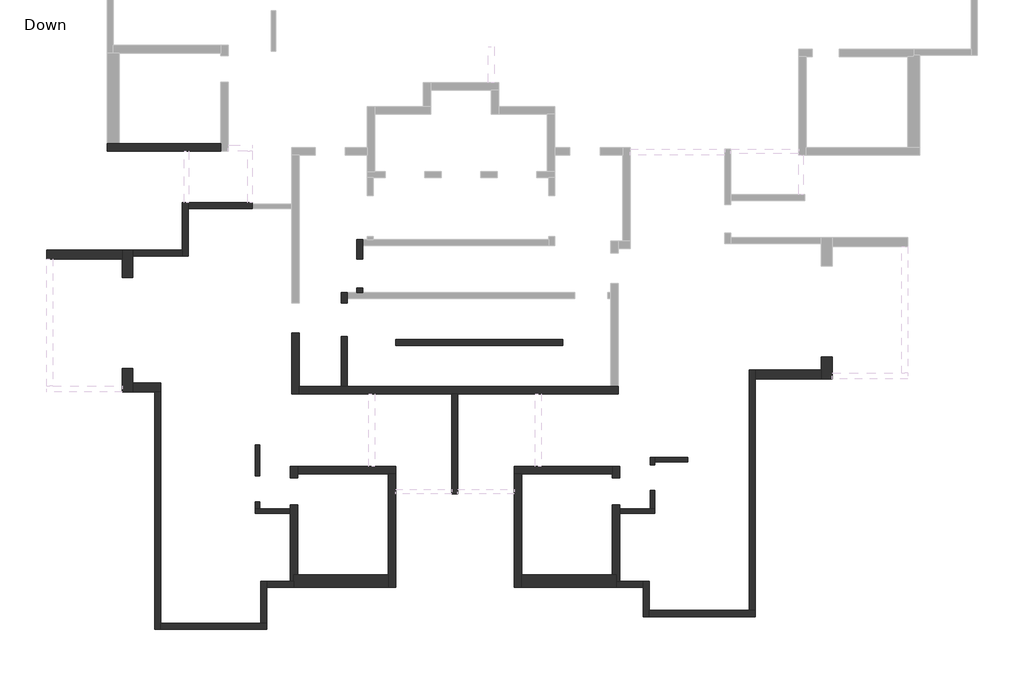
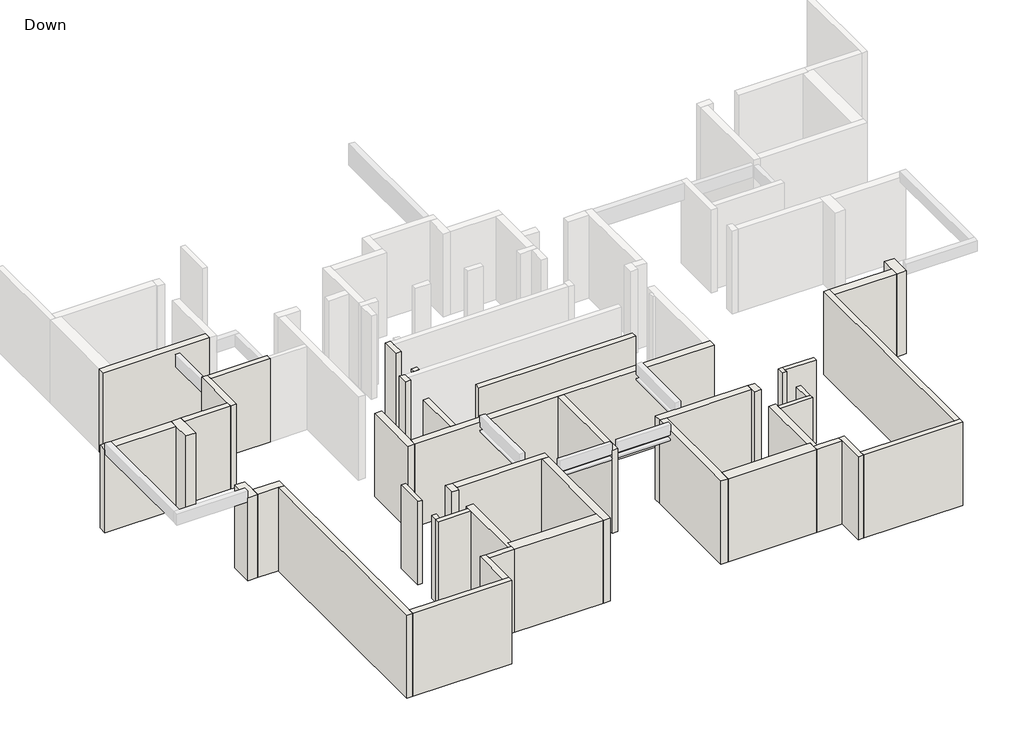
# One storey, part 1 of 3: 43 walls.
"""IFC4 building model written with IfcOpenShell, lengths in millimetres."""

import ifcopenshell
import ifcopenshell.guid

model = None  # the IFC model being written
_history = None  # IfcOwnerHistory: only IFC2X3 demands one
_inside = {}  # id of a spatial element -> (the spatial element, [elements in it])
_under = {}  # id of a project, library or spatial element -> (it, [spatial elements below it])
_declared = {}  # id of a project -> (the project, [libraries it declares])
_typed = {}  # id of a type object -> (the type object, [elements of that type])
_made_of = {}  # id of a material, layer set ... -> (it, [elements and type objects made of it])


def new_model(schema):
    """Start an empty IFC model of exactly this schema.

    Asked for "IFC4X3", IfcOpenShell would pick the latest addendum, in which some entities
    have other attributes; the version numbers below select the first issue.
    IFC2X3 requires an IfcOwnerHistory on every rooted entity: one is made here for all.
    """
    global model, _history
    if schema == "IFC4X3":
        model = ifcopenshell.file(schema_version=(4, 3, 0, 0))
    else:
        model = ifcopenshell.file(schema=schema)
    _inside.clear()
    _under.clear()
    _declared.clear()
    _typed.clear()
    _made_of.clear()
    _history = None
    if model.schema == "IFC2X3":
        org = make("IfcOrganization", Name="unknown")
        user = make(
            "IfcPersonAndOrganization",
            ThePerson=make("IfcPerson", FamilyName="unknown"),
            TheOrganization=org,
        )
        app = make(
            "IfcApplication",
            ApplicationDeveloper=org,
            Version="unknown",
            ApplicationFullName="unknown",
            ApplicationIdentifier="unknown",
        )
        _history = make(
            "IfcOwnerHistory",
            OwningUser=user,
            OwningApplication=app,
            ChangeAction="ADDED",
            CreationDate=0,
        )
    return model


def make(cls, **values):
    """One entity of the class cls with the attributes given. An attribute that is None is left unset."""
    return model.create_entity(
        cls, **{name: value for name, value in values.items() if value is not None}
    )


def rooted(cls, **values):
    """An entity with a GlobalId (a new one), such as an element, a storey or a relation."""
    return make(cls, GlobalId=ifcopenshell.guid.new(), OwnerHistory=_history, **values)


def si_unit(unit_type, name, prefix=None):
    """IfcSIUnit, for example si_unit("LENGTHUNIT", "METRE", prefix="MILLI")."""
    return make("IfcSIUnit", UnitType=unit_type, Prefix=prefix, Name=name)


def assignment(units):
    """IfcUnitAssignment: the units of a project."""
    return None if units is None else make("IfcUnitAssignment", Units=units)


def point(xyz):
    """IfcCartesianPoint."""
    return None if xyz is None else make("IfcCartesianPoint", Coordinates=xyz)


def direction(xyz):
    """IfcDirection."""
    return None if xyz is None else make("IfcDirection", DirectionRatios=xyz)


def frame(location, z_axis=None, x_axis=None):
    """IfcAxis2Placement3D, a coordinate frame: its origin and axes. An axis left out is left unset."""
    return make(
        "IfcAxis2Placement3D",
        Location=point(location),
        Axis=direction(z_axis),
        RefDirection=direction(x_axis),
    )


def origin():
    """The frame at (0, 0, 0) with its axes left unset."""
    return frame((0.0, 0.0, 0.0))


def place(relative_to, where):
    """IfcLocalPlacement: puts the frame where relative to a parent placement (None: the world)."""
    return make(
        "IfcLocalPlacement", PlacementRelTo=relative_to, RelativePlacement=where
    )


def context(
    kind, dimensions, precision=None, world=None, true_north=None, identifier=None
):
    """IfcGeometricRepresentationContext, for example the 3D "Model" context."""
    return make(
        "IfcGeometricRepresentationContext",
        ContextIdentifier=identifier,
        ContextType=kind,
        CoordinateSpaceDimension=dimensions,
        Precision=precision,
        WorldCoordinateSystem=world,
        TrueNorth=true_north,
    )


def project(units=None, contexts=None):
    """IfcProject with its units and contexts."""
    return rooted(
        "IfcProject",
        Name="project",
        RepresentationContexts=contexts,
        UnitsInContext=assignment(units),
    )


def spatial(cls, under=None, at=None, **own):
    """A site, building, storey or space (cls), placed at a placement, below another one or the project."""
    s = rooted(cls, ObjectPlacement=at, **own)
    if under is not None:
        _under.setdefault(under.id(), (under, []))[1].append(s)
    return s


def faces_of(points, faces, orient=None, outer=None):
    """IfcFace entities. A face is a list of loops; a loop is a list of indices into points, from 0.

    orient and outer hold one flag for each loop. By default every Orientation is true, the
    first loop of a face is its IfcFaceOuterBound and the others are IfcFaceBound.
    """
    made = []
    for i, loops in enumerate(faces):
        bounds = []
        for j, loop in enumerate(loops):
            is_outer = j == 0 if outer is None else outer[i][j]
            bounds.append(
                make(
                    "IfcFaceOuterBound" if is_outer else "IfcFaceBound",
                    Bound=make("IfcPolyLoop", Polygon=[points[k] for k in loop]),
                    Orientation=True if orient is None else orient[i][j],
                )
            )
        made.append(make("IfcFace", Bounds=bounds))
    return made


def faceted_brep(points, faces, orient=None, outer=None, voids=None):
    """IfcFacetedBrep: a solid bounded by flat faces; with voids (closed shells), ...WithVoids."""
    shared = [point(p) for p in points]
    hull = make("IfcClosedShell", CfsFaces=faces_of(shared, faces, orient, outer))
    if voids is None:
        return make("IfcFacetedBrep", Outer=hull)
    return make(
        "IfcFacetedBrepWithVoids",
        Outer=hull,
        Voids=[
            make(cls, CfsFaces=faces_of(shared, fs, o, b)) for cls, fs, o, b in voids
        ],
    )


def shape(context_of_items, identifier, shape_type, items):
    """IfcShapeRepresentation: the items that make up one representation, for example the "Body"."""
    return make(
        "IfcShapeRepresentation",
        ContextOfItems=context_of_items,
        RepresentationIdentifier=identifier,
        RepresentationType=shape_type,
        Items=items,
    )


def made_of(thing, what):
    """Note that an element or type object is made of a material, layer set ...; save() writes the relation."""
    if what is not None:
        _made_of.setdefault(what.id(), (what, []))[1].append(thing)
    return thing


def element(
    cls,
    number,
    at=None,
    inside=None,
    cuts=None,
    type_object=None,
    material=None,
    context=None,
    identifier="Body",
    shape_type=None,
    held_by="IfcProductDefinitionShape",
    body=None,
    shapes=None,
    **own,
):
    """One element of the class cls, such as IfcWall. Its Tag is "e" and its number.

    at: its placement. inside: the storey or other place that contains it. cuts: it is an
    opening in that element (IfcRelVoidsElement). A single representation is given by context,
    identifier, shape_type and body (its items); several are given by shapes. held_by: the class
    of the entity that holds the representations. save() writes the other relations.
    """
    e = rooted(cls, Tag="e%d" % number, ObjectPlacement=at, **own)
    if body is not None:
        shapes = [shape(context, identifier, shape_type, body)]
    if shapes is not None:
        e.Representation = make(held_by, Representations=shapes)
    if inside is not None:
        _inside.setdefault(inside.id(), (inside, []))[1].append(e)
    if cuts is not None:
        rooted(
            "IfcRelVoidsElement", RelatingBuildingElement=cuts, RelatedOpeningElement=e
        )
    if type_object is not None:
        _typed.setdefault(type_object.id(), (type_object, []))[1].append(e)
    return made_of(e, material)


def aggregate(whole, parts):
    """IfcRelAggregates: a whole, such as a stair, and the parts it consists of."""
    return rooted("IfcRelAggregates", RelatingObject=whole, RelatedObjects=parts)


def save(model, path):
    """Write the relations noted so far, then the file.

    IfcRelAggregates (storeys below a building ...), IfcRelContainedInSpatialStructure (elements
    in a storey), IfcRelDefinesByType, IfcRelAssociatesMaterial and IfcRelDeclares: one each for
    every whole, place, type object, material and project.
    """
    for whole, parts in _under.values():
        aggregate(whole, parts)
    for where, things in _inside.values():
        rooted(
            "IfcRelContainedInSpatialStructure",
            RelatedElements=things,
            RelatingStructure=where,
        )
    for kind, things in _typed.values():
        rooted("IfcRelDefinesByType", RelatedObjects=things, RelatingType=kind)
    for what, things in _made_of.values():
        rooted("IfcRelAssociatesMaterial", RelatedObjects=things, RelatingMaterial=what)
    for by, libraries in _declared.values():
        rooted("IfcRelDeclares", RelatingContext=by, RelatedDefinitions=libraries)
    model.write(path)


model = new_model("IFC4")

# Units and contexts
model_context = context("Model", 3, world=origin())
ifc_project = project(units=[si_unit("LENGTHUNIT", "METRE", prefix="MILLI")], contexts=[model_context])

# Site, building, storey
site = spatial("IfcSite", under=ifc_project)
building = spatial("IfcBuilding", under=site)
storey = spatial("IfcBuildingStorey", under=building, Name="Down", Elevation=0.0)

# Walls
placement = place(None, origin())
element("IfcWall", 1, ObjectType="15", at=placement, inside=storey, context=model_context, shape_type="Brep", body=[
    faceted_brep([(9202.7157481, -20705.5131366, 0.0), (8200.3527676, -20705.5131366, 0.0), (8050.3527676, -20705.5131366, 0.0), (8050.3527676, -20705.5131366, 3100.0), (8200.3527676, -20705.5131366, 3100.0), (9202.7157481, -20705.5131366, 3100.0), (9202.7157481, -20705.5131366, 2950.0), (9202.7157481, -20705.5131366, 2730.0), (9202.7157481, -20855.5131366, 0.0), (9202.7157481, -20855.5131366, 2730.0), (9202.7157481, -20855.5131366, 2950.0), (9202.7157481, -20855.5131366, 3100.0), (8050.3527676, -20855.5131366, 3100.0), (8050.3527676, -20855.5131366, 2950.0), (8050.3527676, -20855.5131366, 2730.0), (8050.3527676, -20855.5131366, 0.0)], [[[0, 1, 2, 3, 4, 5, 6, 7]], [[8, 9, 10, 11, 12, 13, 14, 15]], [[2, 1, 0, 8, 15]], [[5, 4, 3, 12, 11]], [[0, 7, 6, 5, 11, 10, 9, 8]], [[3, 2, 15, 14, 13, 12]]]),
])
element("IfcWall", 2, ObjectType="15", at=placement, inside=storey, context=model_context, shape_type="Brep", body=[
    faceted_brep([(8200.3527676, -20705.5131366, 0.0), (8200.3527676, -20474.3903326, 0.0), (8200.3527676, -20474.3903326, 2730.0), (8200.3527676, -20474.3903326, 2950.0), (8200.3527676, -20474.3903326, 3100.0), (8200.3527676, -20705.5131366, 3100.0), (8200.3527676, -20705.5131366, 2950.0), (8200.3527676, -20705.5131366, 2730.0), (8050.3527676, -20705.5131366, 0.0), (8050.3527676, -20705.5131366, 3100.0), (8050.3527676, -20474.3903326, 3100.0), (8050.3527676, -20474.3903326, 2950.0), (8050.3527676, -20474.3903326, 2730.0), (8050.3527676, -20474.3903326, 0.0)], [[[0, 1, 2, 3, 4, 5, 6, 7]], [[8, 9, 10, 11, 12, 13]], [[1, 0, 8, 13]], [[4, 3, 2, 1, 13, 12, 11, 10]], [[5, 4, 10, 9]], [[0, 7, 6, 5, 9, 8]]]),
])
element("IfcWall", 3, ObjectType="15", at=placement, inside=storey, context=model_context, shape_type="Brep", body=[
    faceted_brep([(8200.3527676, -19623.2572222, 0.0), (8200.3527676, -18603.3436751, 0.0), (8200.3527676, -18603.3436751, 2730.0), (8200.3527676, -18603.3436751, 2950.0), (8200.3527676, -18603.3436751, 3100.0), (8200.3527676, -19623.2572222, 3100.0), (8200.3527676, -19623.2572222, 2950.0), (8200.3527676, -19623.2572222, 2730.0), (8050.3527676, -19623.2572222, 0.0), (8050.3527676, -19623.2572222, 2730.0), (8050.3527676, -19623.2572222, 2950.0), (8050.3527676, -19623.2572222, 3100.0), (8050.3527676, -18603.3436751, 3100.0), (8050.3527676, -18603.3436751, 2950.0), (8050.3527676, -18603.3436751, 2730.0), (8050.3527676, -18603.3436751, 0.0)], [[[0, 1, 2, 3, 4, 5, 6, 7]], [[8, 9, 10, 11, 12, 13, 14, 15]], [[1, 0, 8, 15]], [[4, 3, 2, 1, 15, 14, 13, 12]], [[5, 4, 12, 11]], [[0, 7, 6, 5, 11, 10, 9, 8]]]),
])
element("IfcWall", 4, ObjectType="15", at=placement, inside=storey, context=model_context, shape_type="Brep", body=[
    faceted_brep([(20111.1907174, -20855.5131366, 0.0), (21263.5536979, -20855.5131366, 0.0), (21263.5536979, -20855.5131366, 2730.0), (21263.5536979, -20855.5131366, 2950.0), (21263.5536979, -20855.5131366, 3100.0), (20111.1907174, -20855.5131366, 3100.0), (20111.1907174, -20855.5131366, 2950.0), (20111.1907174, -20855.5131366, 2730.0), (20111.1907174, -20705.5131366, 0.0), (20111.1907174, -20705.5131366, 2730.0), (20111.1907174, -20705.5131366, 2950.0), (20111.1907174, -20705.5131366, 3100.0), (21113.5536979, -20705.5131366, 3100.0), (21263.5536979, -20705.5131366, 3100.0), (21263.5536979, -20705.5131366, 0.0), (21113.5536979, -20705.5131366, 0.0)], [[[0, 1, 2, 3, 4, 5, 6, 7]], [[8, 9, 10, 11, 12, 13, 14, 15]], [[1, 0, 8, 15, 14]], [[5, 4, 13, 12, 11]], [[0, 7, 6, 5, 11, 10, 9, 8]], [[4, 3, 2, 1, 14, 13]]]),
])
element("IfcWall", 5, ObjectType="15", at=placement, inside=storey, context=model_context, shape_type="Brep", body=[
    faceted_brep([(21263.5536979, -20705.5131366, 0.0), (21263.5536979, -20105.5131366, 0.0), (21263.5536979, -20105.5131366, 2730.0), (21263.5536979, -20105.5131366, 2950.0), (21263.5536979, -20105.5131366, 3100.0), (21263.5536979, -20705.5131366, 3100.0), (21113.5536979, -20705.5131366, 0.0), (21113.5536979, -20705.5131366, 2730.0), (21113.5536979, -20705.5131366, 2950.0), (21113.5536979, -20705.5131366, 3100.0), (21113.5536979, -20105.5131366, 3100.0), (21113.5536979, -20105.5131366, 2950.0), (21113.5536979, -20105.5131366, 2730.0), (21113.5536979, -20105.5131366, 0.0)], [[[0, 1, 2, 3, 4, 5]], [[6, 7, 8, 9, 10, 11, 12, 13]], [[1, 0, 6, 13]], [[4, 3, 2, 1, 13, 12, 11, 10]], [[5, 4, 10, 9]], [[0, 5, 9, 8, 7, 6]]]),
])
element("IfcWall", 6, ObjectType="15", at=placement, inside=storey, context=model_context, shape_type="Brep", body=[
    faceted_brep([(21258.5265415, -19255.7144534, 0.0), (21258.5265415, -19155.8065343, 0.0), (21258.5265415, -19005.8065343, 0.0), (21258.5265415, -19005.8065343, 3100.0), (21258.5265415, -19155.8065343, 3100.0), (21258.5265415, -19255.7144534, 3100.0), (21258.5265415, -19255.7144534, 2950.0), (21258.5265415, -19255.7144534, 2730.0), (21108.5265415, -19255.7144534, 0.0), (21108.5265415, -19255.7144534, 2730.0), (21108.5265415, -19255.7144534, 2950.0), (21108.5265415, -19255.7144534, 3100.0), (21108.5265415, -19005.8065343, 3100.0), (21108.5265415, -19005.8065343, 2950.0), (21108.5265415, -19005.8065343, 2730.0), (21108.5265415, -19005.8065343, 0.0)], [[[0, 1, 2, 3, 4, 5, 6, 7]], [[8, 9, 10, 11, 12, 13, 14, 15]], [[2, 1, 0, 8, 15]], [[5, 4, 3, 12, 11]], [[0, 7, 6, 5, 11, 10, 9, 8]], [[3, 2, 15, 14, 13, 12]]]),
])
element("IfcWall", 7, ObjectType="15", at=placement, inside=storey, context=model_context, shape_type="Brep", body=[
    faceted_brep([(21258.5265415, -19155.8065343, 0.0), (22357.1843165, -19155.8065343, 0.0), (22357.1843165, -19155.8065343, 2730.0), (22357.1843165, -19155.8065343, 2950.0), (22357.1843165, -19155.8065343, 3100.0), (21258.5265415, -19155.8065343, 3100.0), (21258.5265415, -19155.8065343, 2950.0), (21258.5265415, -19155.8065343, 2730.0), (21258.5265415, -19005.8065343, 0.0), (21258.5265415, -19005.8065343, 3100.0), (22357.1843165, -19005.8065343, 3100.0), (22357.1843165, -19005.8065343, 2950.0), (22357.1843165, -19005.8065343, 2730.0), (22357.1843165, -19005.8065343, 0.0)], [[[0, 1, 2, 3, 4, 5, 6, 7]], [[8, 9, 10, 11, 12, 13]], [[1, 0, 8, 13]], [[4, 3, 2, 1, 13, 12, 11, 10]], [[5, 4, 10, 9]], [[0, 7, 6, 5, 9, 8]]]),
])
element("IfcWall", 8, ObjectType="20", at=placement, inside=storey, context=model_context, shape_type="Brep", body=[
    faceted_brep([(4004.7368494, -12353.0033555, 0.0), (5645.6252471, -12353.0033555, 0.0), (5645.6252471, -12353.0033555, 3100.0), (4004.7368494, -12353.0033555, 3100.0), (4004.7368494, -12353.0033555, 2950.0), (4004.7368494, -12353.0033555, 2730.0), (4004.7368494, -12153.0033555, 0.0), (4004.7368494, -12153.0033555, 3100.0), (5645.6252471, -12153.0033555, 3100.0), (5645.6252471, -12153.0033555, 0.0)], [[[0, 1, 2, 3, 4, 5]], [[6, 7, 8, 9]], [[1, 0, 6, 9]], [[3, 2, 8, 7]], [[2, 1, 9, 8]], [[0, 5, 4, 3, 7, 6]]]),
])
element("IfcWall", 9, ObjectType="20", at=placement, inside=storey, context=model_context, shape_type="Brep", body=[
    faceted_brep([(5845.6252471, -12353.0033555, 0.0), (5845.6252471, -10774.5447275, 0.0), (5845.6252471, -10574.5447275, 0.0), (5845.6252471, -10574.5447275, 3100.0), (5845.6252471, -10774.5447275, 3100.0), (5845.6252471, -12353.0033555, 3100.0), (5845.6252471, -12353.0033555, 2950.0), (5845.6252471, -12353.0033555, 2730.0), (5645.6252471, -12353.0033555, 0.0), (5645.6252471, -12353.0033555, 3100.0), (5645.6252471, -12153.0033555, 3100.0), (5645.6252471, -10574.5447275, 3100.0), (5645.6252471, -10574.5447275, 0.0), (5645.6252471, -12153.0033555, 0.0)], [[[0, 1, 2, 3, 4, 5, 6, 7]], [[8, 9, 10, 11, 12, 13]], [[2, 1, 0, 8, 13, 12]], [[5, 4, 3, 11, 10, 9]], [[0, 7, 6, 5, 9, 8]], [[3, 2, 12, 11]]]),
])
element("IfcWall", 10, ObjectType="20", at=placement, inside=storey, context=model_context, shape_type="Brep", body=[
    faceted_brep([(5845.6252471, -10774.5447275, 0.0), (7954.0579731, -10774.5447275, 0.0), (7954.0579731, -10774.5447275, 3100.0), (5845.6252471, -10774.5447275, 3100.0), (5845.6252471, -10774.5447275, 2950.0), (5845.6252471, -10774.5447275, 2730.0), (5845.6252471, -10574.5447275, 0.0), (5845.6252471, -10574.5447275, 3100.0), (7954.0579731, -10574.5447275, 3100.0), (7954.0579731, -10574.5447275, 2450.0), (7954.0579731, -10574.5447275, 2300.0), (7954.0579731, -10574.5447275, 0.0), (7954.0579731, -10624.5447275, 0.0), (7954.0579731, -10624.5447275, 3100.0)], [[[0, 1, 2, 3, 4, 5]], [[6, 7, 8, 9, 10, 11]], [[1, 0, 6, 11, 12]], [[2, 1, 12, 11, 10, 9, 8, 13]], [[3, 2, 13, 8, 7]], [[0, 5, 4, 3, 7, 6]]]),
])
element("IfcWall", 11, ObjectType="20", at=placement, inside=storey, context=model_context, shape_type="Brep", body=[
    faceted_brep([(4732.0592479, -16842.3482114, 0.0), (4732.0592479, -24693.724882, 0.0), (4732.0592479, -24693.724882, 3100.0), (4732.0592479, -16842.3482114, 3100.0), (4932.0592479, -16842.3482114, 0.0), (4932.0592479, -16842.3482114, 3100.0), (4932.0592479, -24493.724882, 3100.0), (4932.0592479, -24693.724882, 3100.0), (4932.0592479, -24693.724882, 0.0), (4932.0592479, -24493.724882, 0.0)], [[[0, 1, 2, 3]], [[4, 5, 6, 7, 8, 9]], [[1, 0, 4, 9, 8]], [[3, 2, 7, 6, 5]], [[2, 1, 8, 7]], [[0, 3, 5, 4]]]),
])
element("IfcWall", 12, ObjectType="20", at=placement, inside=storey, context=model_context, shape_type="Brep", body=[
    faceted_brep([(4932.0592479, -24693.724882, 0.0), (8431.4755716, -24693.724882, 0.0), (8431.4755716, -24693.724882, 3100.0), (4932.0592479, -24693.724882, 3100.0), (4932.0592479, -24493.724882, 0.0), (4932.0592479, -24493.724882, 2730.0), (4932.0592479, -24493.724882, 2950.0), (4932.0592479, -24493.724882, 3100.0), (8231.4755716, -24493.724882, 3100.0), (8431.4755716, -24493.724882, 3100.0), (8431.4755716, -24493.724882, 0.0), (8231.4755716, -24493.724882, 0.0)], [[[0, 1, 2, 3]], [[4, 5, 6, 7, 8, 9, 10, 11]], [[1, 0, 4, 11, 10]], [[3, 2, 9, 8, 7]], [[0, 3, 7, 6, 5, 4]], [[2, 1, 10, 9]]]),
])
element("IfcWall", 13, ObjectType="20", at=placement, inside=storey, context=model_context, shape_type="Brep", body=[
    faceted_brep([(8431.4755716, -24493.724882, 0.0), (8431.4755716, -23302.7444034, 0.0), (8431.4755716, -23102.7444034, 0.0), (8431.4755716, -23102.7444034, 3100.0), (8431.4755716, -23302.7444034, 3100.0), (8431.4755716, -24493.724882, 3100.0), (8231.4755716, -24493.724882, 0.0), (8231.4755716, -24493.724882, 2730.0), (8231.4755716, -24493.724882, 2950.0), (8231.4755716, -24493.724882, 3100.0), (8231.4755716, -23102.7444034, 3100.0), (8231.4755716, -23102.7444034, 2950.0), (8231.4755716, -23102.7444034, 2730.0), (8231.4755716, -23102.7444034, 0.0)], [[[0, 1, 2, 3, 4, 5]], [[6, 7, 8, 9, 10, 11, 12, 13]], [[2, 1, 0, 6, 13]], [[5, 4, 3, 10, 9]], [[0, 5, 9, 8, 7, 6]], [[3, 2, 13, 12, 11, 10]]]),
])
element("IfcWall", 14, ObjectType="20", at=placement, inside=storey, context=model_context, shape_type="Brep", body=[
    faceted_brep([(8431.4755716, -23302.7444034, 0.0), (9327.7157481, -23302.7444034, 0.0), (9327.7157481, -23302.7444034, 3100.0), (8431.4755716, -23302.7444034, 3100.0), (8431.4755716, -23102.7444034, 0.0), (8431.4755716, -23102.7444034, 3100.0), (9202.7157481, -23102.7444034, 3100.0), (9327.7157481, -23102.7444034, 3100.0), (9327.7157481, -23102.7444034, 0.0), (9202.7157481, -23102.7444034, 0.0)], [[[0, 1, 2, 3]], [[4, 5, 6, 7, 8, 9]], [[1, 0, 4, 9, 8]], [[2, 1, 8, 7]], [[3, 2, 7, 6, 5]], [[0, 3, 5, 4]]]),
])
element("IfcWall", 15, ObjectType="20", at=placement, inside=storey, context=model_context, shape_type="Brep", body=[
    faceted_brep([(14756.9532328, -20224.3060494, 0.0), (14756.9532328, -16906.0156488, 0.0), (14756.9532328, -16906.0156488, 2800.0), (14756.9532328, -16906.0156488, 2950.0), (14756.9532328, -16906.0156488, 3100.0), (14756.9532328, -20224.3060494, 3100.0), (14756.9532328, -20224.3060494, 2950.0), (14756.9532328, -20224.3060494, 2800.0), (14756.9532328, -20224.3060494, 2750.0), (14556.9532328, -20224.3060494, 0.0), (14556.9532328, -20224.3060494, 2750.0), (14556.9532328, -20224.3060494, 2800.0), (14556.9532328, -20224.3060494, 2950.0), (14556.9532328, -20224.3060494, 3100.0), (14556.9532328, -16906.0156488, 3100.0), (14556.9532328, -16906.0156488, 2950.0), (14556.9532328, -16906.0156488, 2800.0), (14556.9532328, -16906.0156488, 0.0)], [[[0, 1, 2, 3, 4, 5, 6, 7, 8]], [[9, 10, 11, 12, 13, 14, 15, 16, 17]], [[1, 0, 9, 17]], [[5, 4, 14, 13]], [[0, 8, 7, 6, 5, 13, 12, 11, 10, 9]], [[4, 3, 2, 1, 17, 16, 15, 14]]]),
])
element("IfcWall", 16, ObjectType="20", at=placement, inside=storey, context=model_context, shape_type="Brep", body=[
    faceted_brep([(21082.430894, -24277.7444034, 0.0), (21082.430894, -24077.7444034, 0.0), (21082.430894, -23102.7444034, 0.0), (21082.430894, -23102.7444034, 2730.0), (21082.430894, -23102.7444034, 2950.0), (21082.430894, -23102.7444034, 3100.0), (21082.430894, -24077.7444034, 3100.0), (21082.430894, -24277.7444034, 3100.0), (20882.430894, -24277.7444034, 0.0), (20882.430894, -24277.7444034, 3100.0), (20882.430894, -23302.7444034, 3100.0), (20882.430894, -23102.7444034, 3100.0), (20882.430894, -23102.7444034, 0.0), (20882.430894, -23302.7444034, 0.0)], [[[0, 1, 2, 3, 4, 5, 6, 7]], [[8, 9, 10, 11, 12, 13]], [[2, 1, 0, 8, 13, 12]], [[7, 6, 5, 11, 10, 9]], [[5, 4, 3, 2, 12, 11]], [[0, 7, 9, 8]]]),
])
element("IfcWall", 17, ObjectType="20", at=placement, inside=storey, context=model_context, shape_type="Brep", body=[
    faceted_brep([(20882.430894, -23102.7444034, 0.0), (20111.1907174, -23102.7444034, 0.0), (19986.1907174, -23102.7444034, 0.0), (19986.1907174, -23102.7444034, 3100.0), (20111.1907174, -23102.7444034, 3100.0), (20882.430894, -23102.7444034, 3100.0), (20882.430894, -23302.7444034, 0.0), (20882.430894, -23302.7444034, 3100.0), (19986.1907174, -23302.7444034, 3100.0), (19986.1907174, -23302.7444034, 0.0)], [[[0, 1, 2, 3, 4, 5]], [[6, 7, 8, 9]], [[2, 1, 0, 6, 9]], [[3, 2, 9, 8]], [[5, 4, 3, 8, 7]], [[0, 5, 7, 6]]]),
])
element("IfcWall", 18, ObjectType="20", at=placement, inside=storey, context=model_context, shape_type="Brep", body=[
    faceted_brep([(21082.430894, -24277.7444034, 0.0), (24582.430894, -24277.7444034, 0.0), (24582.430894, -24277.7444034, 3100.0), (21082.430894, -24277.7444034, 3100.0), (21082.430894, -24077.7444034, 0.0), (21082.430894, -24077.7444034, 2730.0), (21082.430894, -24077.7444034, 2950.0), (21082.430894, -24077.7444034, 3100.0), (24382.430894, -24077.7444034, 3100.0), (24582.430894, -24077.7444034, 3100.0), (24582.430894, -24077.7444034, 0.0), (24382.430894, -24077.7444034, 0.0)], [[[0, 1, 2, 3]], [[4, 5, 6, 7, 8, 9, 10, 11]], [[1, 0, 4, 11, 10]], [[3, 2, 9, 8, 7]], [[0, 3, 7, 6, 5, 4]], [[2, 1, 10, 9]]]),
])
element("IfcWall", 19, ObjectType="20", at=placement, inside=storey, context=model_context, shape_type="Brep", body=[
    faceted_brep([(24582.430894, -24077.7444034, 0.0), (24582.430894, -16418.7263398, 0.0), (24582.430894, -16118.7263398, 0.0), (24582.430894, -16118.7263398, 3100.0), (24582.430894, -16418.7263398, 3100.0), (24582.430894, -24077.7444034, 3100.0), (24382.430894, -24077.7444034, 0.0), (24382.430894, -24077.7444034, 2730.0), (24382.430894, -24077.7444034, 2950.0), (24382.430894, -24077.7444034, 3100.0), (24382.430894, -16118.7263398, 3100.0), (24382.430894, -16118.7263398, 2950.0), (24382.430894, -16118.7263398, 2730.0), (24382.430894, -16118.7263398, 0.0)], [[[0, 1, 2, 3, 4, 5]], [[6, 7, 8, 9, 10, 11, 12, 13]], [[2, 1, 0, 6, 13]], [[5, 4, 3, 10, 9]], [[0, 5, 9, 8, 7, 6]], [[3, 2, 13, 12, 11, 10]]]),
])
element("IfcWall", 20, ObjectType="20", at=placement, inside=storey, context=model_context, shape_type="Brep", body=[
    faceted_brep([(11403.5632586, -11804.3284255, 0.0), (11403.5632586, -12452.9986769, 0.0), (11403.5632586, -12452.9986769, 2730.0), (11403.5632586, -12452.9986769, 2950.0), (11403.5632586, -12452.9986769, 3100.0), (11403.5632586, -11804.3284255, 3100.0), (11403.5632586, -11804.3284255, 2950.0), (11403.5632586, -11804.3284255, 2730.0), (11603.5632586, -11804.3284255, 0.0), (11603.5632586, -11804.3284255, 3100.0), (11603.5632586, -12004.3284255, 3100.0), (11603.5632586, -12452.9986769, 3100.0), (11603.5632586, -12452.9986769, 2950.0), (11603.5632586, -12452.9986769, 2730.0), (11603.5632586, -12452.9986769, 0.0), (11603.5632586, -12004.3284255, 0.0)], [[[0, 1, 2, 3, 4, 5, 6, 7]], [[8, 9, 10, 11, 12, 13, 14, 15]], [[1, 0, 8, 15, 14]], [[4, 3, 2, 1, 14, 13, 12, 11]], [[5, 4, 11, 10, 9]], [[0, 7, 6, 5, 9, 8]]]),
])
element("IfcWall", 21, ObjectType="20", at=placement, inside=storey, context=model_context, shape_type="Brep", body=[
    faceted_brep([(11403.5632586, -13405.3647765, 0.0), (11403.5632586, -13552.8020387, 0.0), (11403.5632586, -13552.8020387, 2730.0), (11403.5632586, -13552.8020387, 2950.0), (11403.5632586, -13552.8020387, 3100.0), (11403.5632586, -13405.3647765, 3100.0), (11403.5632586, -13405.3647765, 2950.0), (11403.5632586, -13405.3647765, 2730.0), (11603.5632586, -13405.3647765, 0.0), (11603.5632586, -13405.3647765, 2730.0), (11603.5632586, -13405.3647765, 2950.0), (11603.5632586, -13405.3647765, 3100.0), (11603.5632586, -13552.8020387, 3100.0), (11603.5632586, -13552.8020387, 2950.0), (11603.5632586, -13552.8020387, 2730.0), (11603.5632586, -13552.8020387, 0.0)], [[[0, 1, 2, 3, 4, 5, 6, 7]], [[8, 9, 10, 11, 12, 13, 14, 15]], [[1, 0, 8, 15]], [[5, 4, 12, 11]], [[0, 7, 6, 5, 11, 10, 9, 8]], [[4, 3, 2, 1, 15, 14, 13, 12]]]),
])
element("IfcWall", 22, ObjectType="20", at=placement, inside=storey, context=model_context, shape_type="Brep", body=[
    faceted_brep([(10900.0437745, -13552.8020387, 0.0), (10900.0437745, -13905.1806146, 0.0), (10900.0437745, -13905.1806146, 2730.0), (10900.0437745, -13905.1806146, 2950.0), (10900.0437745, -13905.1806146, 3100.0), (10900.0437745, -13552.8020387, 3100.0), (10900.0437745, -13552.8020387, 2950.0), (10900.0437745, -13552.8020387, 2730.0), (11100.0437745, -13552.8020387, 0.0), (11100.0437745, -13552.8020387, 3100.0), (11100.0437745, -13752.8020387, 3100.0), (11100.0437745, -13905.1806146, 3100.0), (11100.0437745, -13905.1806146, 2950.0), (11100.0437745, -13905.1806146, 2730.0), (11100.0437745, -13905.1806146, 0.0), (11100.0437745, -13752.8020387, 0.0)], [[[0, 1, 2, 3, 4, 5, 6, 7]], [[8, 9, 10, 11, 12, 13, 14, 15]], [[1, 0, 8, 15, 14]], [[4, 3, 2, 1, 14, 13, 12, 11]], [[5, 4, 11, 10, 9]], [[0, 7, 6, 5, 9, 8]]]),
])
element("IfcWall", 23, ObjectType="20", at=placement, inside=storey, context=model_context, shape_type="Brep", body=[
    faceted_brep([(10900.0437745, -15005.1634597, 0.0), (10900.0437745, -16656.0156488, 0.0), (10900.0437745, -16656.0156488, 2730.0), (10900.0437745, -16656.0156488, 2950.0), (10900.0437745, -16656.0156488, 3100.0), (10900.0437745, -15005.1634597, 3100.0), (10900.0437745, -15005.1634597, 2950.0), (10900.0437745, -15005.1634597, 2730.0), (11100.0437745, -15005.1634597, 0.0), (11100.0437745, -15005.1634597, 2730.0), (11100.0437745, -15005.1634597, 2950.0), (11100.0437745, -15005.1634597, 3100.0), (11100.0437745, -16656.0156488, 3100.0), (11100.0437745, -16656.0156488, 2950.0), (11100.0437745, -16656.0156488, 2730.0), (11100.0437745, -16656.0156488, 0.0)], [[[0, 1, 2, 3, 4, 5, 6, 7]], [[8, 9, 10, 11, 12, 13, 14, 15]], [[1, 0, 8, 15]], [[5, 4, 12, 11]], [[0, 7, 6, 5, 11, 10, 9, 8]], [[4, 3, 2, 1, 15, 14, 13, 12]]]),
])
element("IfcWall", 24, ObjectType="20", at=placement, inside=storey, context=model_context, shape_type="Brep", body=[
    faceted_brep([(12694.7247799, -15306.2169656, 0.0), (18213.8626911, -15306.2169656, 0.0), (18213.8626911, -15306.2169656, 2730.0), (18213.8626911, -15306.2169656, 2950.0), (18213.8626911, -15306.2169656, 3100.0), (12694.7247799, -15306.2169656, 3100.0), (12694.7247799, -15106.2169656, 0.0), (12694.7247799, -15106.2169656, 3100.0), (18213.8626911, -15106.2169656, 3100.0), (18213.8626911, -15106.2169656, 2950.0), (18213.8626911, -15106.2169656, 2730.0), (18213.8626911, -15106.2169656, 0.0)], [[[0, 1, 2, 3, 4, 5]], [[6, 7, 8, 9, 10, 11]], [[1, 0, 6, 11]], [[4, 3, 2, 1, 11, 10, 9, 8]], [[5, 4, 8, 7]], [[0, 5, 7, 6]]]),
])
element("IfcWall", 25, ObjectType="25", at=placement, inside=storey, context=model_context, shape_type="Brep", body=[
    faceted_brep([(6907.9504595, -8625.9821525, 0.0), (3557.3073849, -8625.9821525, 0.0), (3157.3073849, -8625.9821525, 0.0), (3157.3073849, -8625.9821525, 3100.0), (3557.3073849, -8625.9821525, 3100.0), (6907.9504595, -8625.9821525, 3100.0), (6907.9504595, -8625.9821525, 2950.0), (6907.9504595, -8625.9821525, 2730.0), (6907.9504595, -8875.9821525, 0.0), (6907.9504595, -8875.9821525, 3100.0), (3157.3073849, -8875.9821525, 3100.0), (3157.3073849, -8875.9821525, 0.0)], [[[0, 1, 2, 3, 4, 5, 6, 7]], [[8, 9, 10, 11]], [[2, 1, 0, 8, 11]], [[5, 4, 3, 10, 9]], [[0, 7, 6, 5, 9, 8]], [[3, 2, 11, 10]]]),
])
element("IfcWall", 26, ObjectType="25", at=placement, inside=storey, context=model_context, shape_type="Brep", body=[
    faceted_brep([(9452.7157481, -19695.7428642, 0.0), (9452.7157481, -19551.9218456, 0.0), (9452.7157481, -19301.9218456, 0.0), (9452.7157481, -19301.9218456, 3100.0), (9452.7157481, -19551.9218456, 3100.0), (9452.7157481, -19695.7428642, 3100.0), (9452.7157481, -19695.7428642, 2950.0), (9452.7157481, -19695.7428642, 2730.0), (9202.7157481, -19695.7428642, 0.0), (9202.7157481, -19695.7428642, 2730.0), (9202.7157481, -19695.7428642, 2950.0), (9202.7157481, -19695.7428642, 3100.0), (9202.7157481, -19301.9218456, 3100.0), (9202.7157481, -19301.9218456, 2950.0), (9202.7157481, -19301.9218456, 2730.0), (9202.7157481, -19301.9218456, 0.0)], [[[0, 1, 2, 3, 4, 5, 6, 7]], [[8, 9, 10, 11, 12, 13, 14, 15]], [[2, 1, 0, 8, 15]], [[5, 4, 3, 12, 11]], [[0, 7, 6, 5, 11, 10, 9, 8]], [[3, 2, 15, 14, 13, 12]]]),
])
element("IfcWall", 27, ObjectType="25", at=placement, inside=storey, context=model_context, shape_type="Brep", body=[
    faceted_brep([(9452.7157481, -19551.9218456, 0.0), (12452.1320718, -19551.9218456, 0.0), (12702.1320718, -19551.9218456, 0.0), (12702.1320718, -19551.9218456, 3100.0), (12452.1320718, -19551.9218456, 3100.0), (9452.7157481, -19551.9218456, 3100.0), (9452.7157481, -19551.9218456, 2950.0), (9452.7157481, -19551.9218456, 2730.0), (9452.7157481, -19301.9218456, 0.0), (9452.7157481, -19301.9218456, 3100.0), (12702.1320718, -19301.9218456, 3100.0), (12702.1320718, -19301.9218456, 2950.0), (12702.1320718, -19301.9218456, 2800.0), (12702.1320718, -19301.9218456, 0.0)], [[[0, 1, 2, 3, 4, 5, 6, 7]], [[8, 9, 10, 11, 12, 13]], [[2, 1, 0, 8, 13]], [[5, 4, 3, 10, 9]], [[0, 7, 6, 5, 9, 8]], [[3, 2, 13, 12, 11, 10]]]),
])
element("IfcWall", 28, ObjectType="25", at=placement, inside=storey, context=model_context, shape_type="Brep", body=[
    faceted_brep([(12452.1320718, -19551.9218456, 0.0), (12452.1320718, -22902.7444034, 0.0), (12452.1320718, -23302.7444034, 0.0), (12452.1320718, -23302.7444034, 3100.0), (12452.1320718, -22902.7444034, 3100.0), (12452.1320718, -19551.9218456, 3100.0), (12452.1320718, -19551.9218456, 2950.0), (12452.1320718, -19551.9218456, 2730.0), (12702.1320718, -19551.9218456, 0.0), (12702.1320718, -19551.9218456, 3100.0), (12702.1320718, -23302.7444034, 3100.0), (12702.1320718, -23302.7444034, 0.0)], [[[0, 1, 2, 3, 4, 5, 6, 7]], [[8, 9, 10, 11]], [[2, 1, 0, 8, 11]], [[5, 4, 3, 10, 9]], [[0, 7, 6, 5, 9, 8]], [[3, 2, 11, 10]]]),
])
element("IfcWall", 29, ObjectType="25", at=placement, inside=storey, context=model_context, shape_type="Brep", body=[
    faceted_brep([(9452.7157481, -22902.7444034, 0.0), (9452.7157481, -20584.2651623, 0.0), (9452.7157481, -20584.2651623, 2730.0), (9452.7157481, -20584.2651623, 2950.0), (9452.7157481, -20584.2651623, 3100.0), (9452.7157481, -22902.7444034, 3100.0), (9452.7157481, -22902.7444034, 2950.0), (9452.7157481, -22902.7444034, 2730.0), (9202.7157481, -23102.7444034, 0.0), (9202.7157481, -23102.7444034, 2730.0), (9202.7157481, -23102.7444034, 2950.0), (9202.7157481, -23102.7444034, 3100.0), (9202.7157481, -20855.5131366, 3100.0), (9202.7157481, -20705.5131366, 3100.0), (9202.7157481, -20584.2651623, 3100.0), (9202.7157481, -20584.2651623, 2950.0), (9202.7157481, -20584.2651623, 2730.0), (9202.7157481, -20584.2651623, 0.0), (9202.7157481, -20705.5131366, 0.0), (9202.7157481, -20855.5131366, 0.0), (9327.7157481, -22902.7444034, 0.0), (9327.7157481, -23102.7444034, 0.0), (9327.7157481, -23102.7444034, 3100.0), (9327.7157481, -22902.7444034, 3100.0)], [[[0, 1, 2, 3, 4, 5, 6, 7]], [[8, 9, 10, 11, 12, 13, 14, 15, 16, 17, 18, 19]], [[1, 0, 20, 21, 8, 19, 18, 17]], [[4, 3, 2, 1, 17, 16, 15, 14]], [[5, 4, 14, 13, 12, 11, 22, 23]], [[0, 7, 6, 5, 23, 20]], [[23, 22, 21, 20]], [[22, 11, 10, 9, 8, 21]]]),
])
element("IfcWall", 30, ObjectType="25", at=placement, inside=storey, context=model_context, shape_type="Brep", body=[
    faceted_brep([(9252.7110695, -14895.1122659, 0.0), (9252.7110695, -16906.0156488, 0.0), (9252.7110695, -16906.0156488, 2730.0), (9252.7110695, -16906.0156488, 2950.0), (9252.7110695, -16906.0156488, 3100.0), (9252.7110695, -14895.1122659, 3100.0), (9502.7110695, -14895.1122659, 0.0), (9502.7110695, -14895.1122659, 3100.0), (9502.7110695, -16656.0156488, 3100.0), (9502.7110695, -16906.0156488, 3100.0), (9502.7110695, -16906.0156488, 0.0), (9502.7110695, -16656.0156488, 0.0)], [[[0, 1, 2, 3, 4, 5]], [[6, 7, 8, 9, 10, 11]], [[1, 0, 6, 11, 10]], [[5, 4, 9, 8, 7]], [[0, 5, 7, 6]], [[4, 3, 2, 1, 10, 9]]]),
])
element("IfcWall", 31, ObjectType="25", at=placement, inside=storey, context=model_context, shape_type="Brep", body=[
    faceted_brep([(9502.7110695, -16906.0156488, 0.0), (14556.9532328, -16906.0156488, 0.0), (14756.9532328, -16906.0156488, 0.0), (20058.6310988, -16906.0156488, 0.0), (20058.6310988, -16906.0156488, 3100.0), (14756.9532328, -16906.0156488, 3100.0), (14556.9532328, -16906.0156488, 3100.0), (9502.7110695, -16906.0156488, 3100.0), (9502.7110695, -16656.0156488, 0.0), (9502.7110695, -16656.0156488, 3100.0), (10900.0437745, -16656.0156488, 3100.0), (11100.0437745, -16656.0156488, 3100.0), (19808.6310988, -16656.0156488, 3100.0), (20058.6310988, -16656.0156488, 3100.0), (20058.6310988, -16656.0156488, 0.0), (19808.6310988, -16656.0156488, 0.0), (11100.0437745, -16656.0156488, 0.0), (10900.0437745, -16656.0156488, 0.0)], [[[0, 1, 2, 3, 4, 5, 6, 7]], [[8, 9, 10, 11, 12, 13, 14, 15, 16, 17]], [[3, 2, 1, 0, 8, 17, 16, 15, 14]], [[7, 6, 5, 4, 13, 12, 11, 10, 9]], [[0, 7, 9, 8]], [[4, 3, 14, 13]]]),
])
element("IfcWall", 32, ObjectType="25", at=placement, inside=storey, context=model_context, shape_type="Brep", body=[
    faceted_brep([(20111.1907174, -19695.7428642, 0.0), (20111.1907174, -19301.9218456, 0.0), (20111.1907174, -19301.9218456, 2730.0), (20111.1907174, -19301.9218456, 2950.0), (20111.1907174, -19301.9218456, 3100.0), (20111.1907174, -19695.7428642, 3100.0), (20111.1907174, -19695.7428642, 2950.0), (20111.1907174, -19695.7428642, 2730.0), (19861.1907174, -19695.7428642, 0.0), (19861.1907174, -19695.7428642, 2730.0), (19861.1907174, -19695.7428642, 2950.0), (19861.1907174, -19695.7428642, 3100.0), (19861.1907174, -19551.9218456, 3100.0), (19861.1907174, -19301.9218456, 3100.0), (19861.1907174, -19301.9218456, 0.0), (19861.1907174, -19551.9218456, 0.0)], [[[0, 1, 2, 3, 4, 5, 6, 7]], [[8, 9, 10, 11, 12, 13, 14, 15]], [[1, 0, 8, 15, 14]], [[5, 4, 13, 12, 11]], [[0, 7, 6, 5, 11, 10, 9, 8]], [[4, 3, 2, 1, 14, 13]]]),
])
element("IfcWall", 33, ObjectType="25", at=placement, inside=storey, context=model_context, shape_type="Brep", body=[
    faceted_brep([(19861.1907174, -19301.9218456, 0.0), (16611.7743938, -19301.9218456, 0.0), (16611.7743938, -19301.9218456, 2800.0), (16611.7743938, -19301.9218456, 2950.0), (16611.7743938, -19301.9218456, 3100.0), (19861.1907174, -19301.9218456, 3100.0), (19861.1907174, -19551.9218456, 0.0), (19861.1907174, -19551.9218456, 2730.0), (19861.1907174, -19551.9218456, 2950.0), (19861.1907174, -19551.9218456, 3100.0), (16861.7743938, -19551.9218456, 3100.0), (16611.7743938, -19551.9218456, 3100.0), (16611.7743938, -19551.9218456, 0.0), (16861.7743938, -19551.9218456, 0.0)], [[[0, 1, 2, 3, 4, 5]], [[6, 7, 8, 9, 10, 11, 12, 13]], [[1, 0, 6, 13, 12]], [[5, 4, 11, 10, 9]], [[0, 5, 9, 8, 7, 6]], [[4, 3, 2, 1, 12, 11]]]),
])
element("IfcWall", 34, ObjectType="25", at=placement, inside=storey, context=model_context, shape_type="Brep", body=[
    faceted_brep([(16611.7743938, -19551.9218456, 0.0), (16611.7743938, -23302.7444034, 0.0), (16611.7743938, -23302.7444034, 3100.0), (16611.7743938, -19551.9218456, 3100.0), (16861.7743938, -19551.9218456, 0.0), (16861.7743938, -19551.9218456, 2730.0), (16861.7743938, -19551.9218456, 2950.0), (16861.7743938, -19551.9218456, 3100.0), (16861.7743938, -22902.7444034, 3100.0), (16861.7743938, -23302.7444034, 3100.0), (16861.7743938, -23302.7444034, 0.0), (16861.7743938, -22902.7444034, 0.0)], [[[0, 1, 2, 3]], [[4, 5, 6, 7, 8, 9, 10, 11]], [[1, 0, 4, 11, 10]], [[3, 2, 9, 8, 7]], [[0, 3, 7, 6, 5, 4]], [[2, 1, 10, 9]]]),
])
element("IfcWall", 35, ObjectType="25", at=placement, inside=storey, context=model_context, shape_type="Brep", body=[
    faceted_brep([(20111.1907174, -23102.7444034, 0.0), (20111.1907174, -20855.5131366, 0.0), (20111.1907174, -20705.5131366, 0.0), (20111.1907174, -20584.2651623, 0.0), (20111.1907174, -20584.2651623, 2730.0), (20111.1907174, -20584.2651623, 2950.0), (20111.1907174, -20584.2651623, 3100.0), (20111.1907174, -20705.5131366, 3100.0), (20111.1907174, -20855.5131366, 3100.0), (20111.1907174, -23102.7444034, 3100.0), (20111.1907174, -23102.7444034, 2950.0), (20111.1907174, -23102.7444034, 2730.0), (19861.1907174, -22902.7444034, 0.0), (19861.1907174, -22902.7444034, 2730.0), (19861.1907174, -22902.7444034, 2950.0), (19861.1907174, -22902.7444034, 3100.0), (19861.1907174, -20584.2651623, 3100.0), (19861.1907174, -20584.2651623, 2950.0), (19861.1907174, -20584.2651623, 2730.0), (19861.1907174, -20584.2651623, 0.0), (19986.1907174, -23102.7444034, 0.0), (19986.1907174, -22902.7444034, 0.0), (19986.1907174, -22902.7444034, 3100.0), (19986.1907174, -23102.7444034, 3100.0)], [[[0, 1, 2, 3, 4, 5, 6, 7, 8, 9, 10, 11]], [[12, 13, 14, 15, 16, 17, 18, 19]], [[3, 2, 1, 0, 20, 21, 12, 19]], [[6, 5, 4, 3, 19, 18, 17, 16]], [[9, 8, 7, 6, 16, 15, 22, 23]], [[0, 11, 10, 9, 23, 20]], [[23, 22, 21, 20]], [[22, 15, 14, 13, 12, 21]]]),
])
element("IfcWall", 36, ObjectType="30", at=placement, inside=storey, context=model_context, shape_type="Brep", body=[
    faceted_brep([(1151.3421966, -12453.0033555, 0.0), (3654.7368494, -12453.0033555, 0.0), (3654.7368494, -12453.0033555, 2730.0), (3654.7368494, -12453.0033555, 2950.0), (3654.7368494, -12453.0033555, 3100.0), (1151.3421966, -12453.0033555, 3100.0), (1151.3421966, -12453.0033555, 2950.0), (1151.3421966, -12453.0033555, 2730.0), (1151.3421966, -12153.0033555, 0.0), (1151.3421966, -12153.0033555, 3100.0), (3654.7368494, -12153.0033555, 3100.0), (3654.7368494, -12153.0033555, 0.0)], [[[0, 1, 2, 3, 4, 5, 6, 7]], [[8, 9, 10, 11]], [[1, 0, 8, 11]], [[5, 4, 10, 9]], [[0, 7, 6, 5, 9, 8]], [[4, 3, 2, 1, 11, 10]]]),
])
element("IfcWall", 37, ObjectType="30", at=placement, inside=storey, context=model_context, shape_type="Brep", body=[
    faceted_brep([(4004.7368494, -16842.3482114, 0.0), (4732.0592479, -16842.3482114, 0.0), (4932.0592479, -16842.3482114, 0.0), (4932.0592479, -16842.3482114, 3100.0), (4732.0592479, -16842.3482114, 3100.0), (4004.7368494, -16842.3482114, 3100.0), (4004.7368494, -16542.3482114, 0.0), (4004.7368494, -16542.3482114, 2730.0), (4004.7368494, -16542.3482114, 2950.0), (4004.7368494, -16542.3482114, 3100.0), (4932.0592479, -16542.3482114, 3100.0), (4932.0592479, -16542.3482114, 2950.0), (4932.0592479, -16542.3482114, 2730.0), (4932.0592479, -16542.3482114, 0.0)], [[[0, 1, 2, 3, 4, 5]], [[6, 7, 8, 9, 10, 11, 12, 13]], [[2, 1, 0, 6, 13]], [[5, 4, 3, 10, 9]], [[0, 5, 9, 8, 7, 6]], [[3, 2, 13, 12, 11, 10]]]),
])
element("IfcWall", 38, ObjectType="30", at=placement, inside=storey, context=model_context, shape_type="Brep", body=[
    faceted_brep([(24582.430894, -16418.7263398, 0.0), (26777.656655, -16418.7263398, 0.0), (26777.656655, -16418.7263398, 3100.0), (24582.430894, -16418.7263398, 3100.0), (24582.430894, -16118.7263398, 0.0), (24582.430894, -16118.7263398, 3100.0), (26777.656655, -16118.7263398, 3100.0), (26777.656655, -16118.7263398, 2950.0), (26777.656655, -16118.7263398, 2730.0), (26777.656655, -16118.7263398, 0.0)], [[[0, 1, 2, 3]], [[4, 5, 6, 7, 8, 9]], [[1, 0, 4, 9]], [[3, 2, 6, 5]], [[0, 3, 5, 4]], [[2, 1, 9, 8, 7, 6]]]),
])
element("IfcWall", 39, ObjectType="35", at=placement, inside=storey, context=model_context, shape_type="Brep", body=[
    faceted_brep([(3654.7368494, -12153.0033555, 0.0), (3654.7368494, -12453.0033555, 0.0), (3654.7368494, -13054.0475042, 0.0), (3654.7368494, -13054.0475042, 2730.0), (3654.7368494, -13054.0475042, 2950.0), (3654.7368494, -13054.0475042, 3100.0), (3654.7368494, -12453.0033555, 3100.0), (3654.7368494, -12153.0033555, 3100.0), (4004.7368494, -12153.0033555, 0.0), (4004.7368494, -12153.0033555, 3100.0), (4004.7368494, -12353.0033555, 3100.0), (4004.7368494, -13054.0475042, 3100.0), (4004.7368494, -13054.0475042, 2950.0), (4004.7368494, -13054.0475042, 2730.0), (4004.7368494, -13054.0475042, 0.0), (4004.7368494, -12353.0033555, 0.0)], [[[0, 1, 2, 3, 4, 5, 6, 7]], [[8, 9, 10, 11, 12, 13, 14, 15]], [[2, 1, 0, 8, 15, 14]], [[5, 4, 3, 2, 14, 13, 12, 11]], [[7, 6, 5, 11, 10, 9]], [[0, 7, 9, 8]]]),
])
element("IfcWall", 40, ObjectType="35", at=placement, inside=storey, context=model_context, shape_type="Brep", body=[
    faceted_brep([(3654.7368494, -16059.997097, 0.0), (3654.7368494, -16842.3482114, 0.0), (3654.7368494, -16842.3482114, 2730.0), (3654.7368494, -16842.3482114, 2950.0), (3654.7368494, -16842.3482114, 3100.0), (3654.7368494, -16059.997097, 3100.0), (3654.7368494, -16059.997097, 2950.0), (3654.7368494, -16059.997097, 2730.0), (4004.7368494, -16059.997097, 0.0), (4004.7368494, -16059.997097, 2730.0), (4004.7368494, -16059.997097, 2950.0), (4004.7368494, -16059.997097, 3100.0), (4004.7368494, -16542.3482114, 3100.0), (4004.7368494, -16842.3482114, 3100.0), (4004.7368494, -16842.3482114, 0.0), (4004.7368494, -16542.3482114, 0.0)], [[[0, 1, 2, 3, 4, 5, 6, 7]], [[8, 9, 10, 11, 12, 13, 14, 15]], [[1, 0, 8, 15, 14]], [[5, 4, 13, 12, 11]], [[0, 7, 6, 5, 11, 10, 9, 8]], [[4, 3, 2, 1, 14, 13]]]),
])
element("IfcWall", 41, ObjectType="35", at=placement, inside=storey, context=model_context, shape_type="Brep", body=[
    faceted_brep([(27127.656655, -16418.7263398, 0.0), (27127.656655, -15678.697929, 0.0), (27127.656655, -15678.697929, 2730.0), (27127.656655, -15678.697929, 2950.0), (27127.656655, -15678.697929, 3100.0), (27127.656655, -16418.7263398, 3100.0), (27127.656655, -16418.7263398, 2950.0), (27127.656655, -16418.7263398, 2730.0), (26777.656655, -16418.7263398, 0.0), (26777.656655, -16418.7263398, 3100.0), (26777.656655, -16118.7263398, 3100.0), (26777.656655, -15678.697929, 3100.0), (26777.656655, -15678.697929, 2950.0), (26777.656655, -15678.697929, 2730.0), (26777.656655, -15678.697929, 0.0), (26777.656655, -16118.7263398, 0.0)], [[[0, 1, 2, 3, 4, 5, 6, 7]], [[8, 9, 10, 11, 12, 13, 14, 15]], [[1, 0, 8, 15, 14]], [[4, 3, 2, 1, 14, 13, 12, 11]], [[5, 4, 11, 10, 9]], [[0, 7, 6, 5, 9, 8]]]),
])
element("IfcWall", 42, ObjectType="40", at=placement, inside=storey, context=model_context, shape_type="Brep", body=[
    faceted_brep([(12452.1320718, -22902.7444034, 0.0), (9452.7157481, -22902.7444034, 0.0), (9327.7157481, -22902.7444034, 0.0), (9327.7157481, -22902.7444034, 3100.0), (9452.7157481, -22902.7444034, 3100.0), (12452.1320718, -22902.7444034, 3100.0), (12452.1320718, -22902.7444034, 2950.0), (12452.1320718, -22902.7444034, 2730.0), (12452.1320718, -23302.7444034, 0.0), (12452.1320718, -23302.7444034, 3100.0), (9327.7157481, -23302.7444034, 3100.0), (9327.7157481, -23302.7444034, 0.0), (9327.7157481, -23102.7444034, 0.0), (9327.7157481, -23102.7444034, 3100.0)], [[[0, 1, 2, 3, 4, 5, 6, 7]], [[8, 9, 10, 11]], [[2, 1, 0, 8, 11, 12]], [[3, 2, 12, 11, 10, 13]], [[5, 4, 3, 13, 10, 9]], [[0, 7, 6, 5, 9, 8]]]),
])
element("IfcWall", 43, ObjectType="40", at=placement, inside=storey, context=model_context, shape_type="Brep", body=[
    faceted_brep([(16861.7743938, -23302.7444034, 0.0), (19986.1907174, -23302.7444034, 0.0), (19986.1907174, -23302.7444034, 3100.0), (16861.7743938, -23302.7444034, 3100.0), (16861.7743938, -22902.7444034, 0.0), (16861.7743938, -22902.7444034, 2730.0), (16861.7743938, -22902.7444034, 2950.0), (16861.7743938, -22902.7444034, 3100.0), (19861.1907174, -22902.7444034, 3100.0), (19986.1907174, -22902.7444034, 3100.0), (19986.1907174, -22902.7444034, 0.0), (19861.1907174, -22902.7444034, 0.0), (19986.1907174, -23102.7444034, 0.0), (19986.1907174, -23102.7444034, 3100.0)], [[[0, 1, 2, 3]], [[4, 5, 6, 7, 8, 9, 10, 11]], [[1, 0, 4, 11, 10, 12]], [[2, 1, 12, 10, 9, 13]], [[3, 2, 13, 9, 8, 7]], [[0, 3, 7, 6, 5, 4]]]),
])

save(model, "model.ifc")

# Revit data of these elements
# Project information
#   Project Issue Date = "Issue Date"
#   Project Status = "Project Status"
#   Client Name = "לקוח"
#   Project Address = "Enter address here"
#   Project Name = "Project 013"
#   Project Number = "מספר פרויקט"
# Type "15"
#   Layers, outside or top first: 15 cm "Concrete" (function 1)
# Type "20"
#   Layers, outside or top first: 20 cm "Concrete" (function 1)
# Type "25"
#   Layers, outside or top first: 25 cm "Concrete" (function 1)
# Type "30"
#   Layers, outside or top first: 30 cm "Concrete" (function 1)
# Type "35"
#   Layers, outside or top first: 35 cm "Concrete" (function 1)
# Type "40"
#   Layers, outside or top first: 40 cm "Concrete" (function 1)
# Element 1 (IfcWall, "15")
#   Comments = ""
#   Mark = "W103"
#   SOFiSTiK_EdgeZones = "W107"
#   SOFiSTiK_AMG_Comments = ""
#   Top Offset = 0 cm
#   Base Offset = 0 cm
#   wall height = 310 cm
#   SOFiSTiK_AMG_Scheduled = yes
#   SOFiSTiK_AMG_Adjusted = yes
#   Phase Created = New Construction
#   Base Constraint = Down
#   Top Constraint = Typical Floor
#   Materials on its faces: "Concrete"
# Element 2 (IfcWall, "15")
#   Comments = ""
#   Mark = "W104"
#   SOFiSTiK_EdgeZones = "W108"
#   SOFiSTiK_AMG_Comments = ""
#   Top Offset = 0 cm
#   Base Offset = 0 cm
#   wall height = 310 cm
#   SOFiSTiK_AMG_Scheduled = yes
#   SOFiSTiK_AMG_Adjusted = yes
#   Phase Created = New Construction
#   Base Constraint = Down
#   Top Constraint = Typical Floor
#   Materials on its faces: "Concrete"
# Element 3 (IfcWall, "15")
#   Comments = ""
#   Mark = "W105"
#   SOFiSTiK_EdgeZones = "W109"
#   SOFiSTiK_AMG_Comments = ""
#   Top Offset = 0 cm
#   Base Offset = 0 cm
#   wall height = 310 cm
#   SOFiSTiK_AMG_Scheduled = yes
#   SOFiSTiK_AMG_Adjusted = yes
#   Phase Created = New Construction
#   Base Constraint = Down
#   Top Constraint = Typical Floor
#   Materials on its faces: "Concrete"
# Element 4 (IfcWall, "15")
#   Comments = ""
#   Mark = "W106"
#   SOFiSTiK_EdgeZones = "W110"
#   SOFiSTiK_AMG_Comments = ""
#   Top Offset = 0 cm
#   Base Offset = 0 cm
#   wall height = 310 cm
#   SOFiSTiK_AMG_Scheduled = yes
#   SOFiSTiK_AMG_Adjusted = yes
#   Phase Created = New Construction
#   Base Constraint = Down
#   Top Constraint = Typical Floor
#   Materials on its faces: "Concrete"
# Element 5 (IfcWall, "15")
#   Comments = ""
#   Mark = "W107"
#   SOFiSTiK_EdgeZones = "W111"
#   SOFiSTiK_AMG_Comments = ""
#   Top Offset = 0 cm
#   Base Offset = 0 cm
#   wall height = 310 cm
#   SOFiSTiK_AMG_Scheduled = yes
#   SOFiSTiK_AMG_Adjusted = yes
#   Phase Created = New Construction
#   Base Constraint = Down
#   Top Constraint = Typical Floor
#   Materials on its faces: "Concrete"
# Element 6 (IfcWall, "15")
#   Comments = ""
#   Mark = "W109"
#   SOFiSTiK_EdgeZones = "W113"
#   SOFiSTiK_AMG_Comments = ""
#   Top Offset = 0 cm
#   Base Offset = 0 cm
#   wall height = 310 cm
#   SOFiSTiK_AMG_Scheduled = yes
#   SOFiSTiK_AMG_Adjusted = yes
#   Phase Created = New Construction
#   Base Constraint = Down
#   Top Constraint = Typical Floor
#   Materials on its faces: "Concrete"
# Element 7 (IfcWall, "15")
#   Comments = ""
#   Mark = "W110"
#   SOFiSTiK_EdgeZones = "W114"
#   SOFiSTiK_AMG_Comments = ""
#   Top Offset = 0 cm
#   Base Offset = 0 cm
#   wall height = 310 cm
#   SOFiSTiK_AMG_Scheduled = yes
#   SOFiSTiK_AMG_Adjusted = yes
#   Phase Created = New Construction
#   Base Constraint = Down
#   Top Constraint = Typical Floor
#   Materials on its faces: "Concrete"
# Element 8 (IfcWall, "20")
#   Comments = ""
#   Mark = "W5"
#   SOFiSTiK_EdgeZones = "W5"
#   SOFiSTiK_AMG_Comments = ""
#   Top Offset = 0 cm
#   Base Offset = 0 cm
#   wall height = 310 cm
#   SOFiSTiK_AMG_Scheduled = yes
#   SOFiSTiK_AMG_Adjusted = yes
#   Phase Created = New Construction
#   Base Constraint = Down
#   Top Constraint = Typical Floor
#   Materials on its faces: "Concrete"
# Element 9 (IfcWall, "20")
#   Comments = ""
#   Mark = "W6"
#   SOFiSTiK_EdgeZones = "W6"
#   SOFiSTiK_AMG_Comments = ""
#   Top Offset = 0 cm
#   Base Offset = 0 cm
#   wall height = 310 cm
#   SOFiSTiK_AMG_Scheduled = yes
#   SOFiSTiK_AMG_Adjusted = yes
#   Phase Created = New Construction
#   Base Constraint = Down
#   Top Constraint = Typical Floor
#   Materials on its faces: "Concrete"
# Element 10 (IfcWall, "20")
#   Comments = ""
#   Mark = "W7"
#   SOFiSTiK_EdgeZones = "W7"
#   SOFiSTiK_AMG_Comments = ""
#   Top Offset = 0 cm
#   Base Offset = 0 cm
#   wall height = 310 cm
#   SOFiSTiK_AMG_Scheduled = yes
#   SOFiSTiK_AMG_Adjusted = yes
#   Phase Created = New Construction
#   Base Constraint = Down
#   Top Constraint = Typical Floor
#   Materials on its faces: "Concrete"
# Element 11 (IfcWall, "20")
#   Comments = ""
#   Mark = "W8"
#   SOFiSTiK_EdgeZones = "W8"
#   SOFiSTiK_AMG_Comments = ""
#   Top Offset = 0 cm
#   Base Offset = 0 cm
#   wall height = 310 cm
#   SOFiSTiK_AMG_Scheduled = yes
#   SOFiSTiK_AMG_Adjusted = yes
#   Phase Created = New Construction
#   Base Constraint = Down
#   Top Constraint = Typical Floor
#   Materials on its faces: "Concrete"
# Element 12 (IfcWall, "20")
#   Comments = ""
#   Mark = "W9"
#   SOFiSTiK_EdgeZones = "W9"
#   SOFiSTiK_AMG_Comments = ""
#   Top Offset = 0 cm
#   Base Offset = 0 cm
#   wall height = 310 cm
#   SOFiSTiK_AMG_Scheduled = yes
#   SOFiSTiK_AMG_Adjusted = yes
#   Phase Created = New Construction
#   Base Constraint = Down
#   Top Constraint = Typical Floor
#   Materials on its faces: "Concrete"
# Element 13 (IfcWall, "20")
#   Comments = ""
#   Mark = "W10"
#   SOFiSTiK_EdgeZones = "W10"
#   SOFiSTiK_AMG_Comments = ""
#   Top Offset = 0 cm
#   Base Offset = 0 cm
#   wall height = 310 cm
#   SOFiSTiK_AMG_Scheduled = yes
#   SOFiSTiK_AMG_Adjusted = yes
#   Phase Created = New Construction
#   Base Constraint = Down
#   Top Constraint = Typical Floor
#   Materials on its faces: "Concrete"
# Element 14 (IfcWall, "20")
#   Comments = ""
#   Mark = "W11"
#   SOFiSTiK_EdgeZones = "W11"
#   SOFiSTiK_AMG_Comments = ""
#   Top Offset = 0 cm
#   Base Offset = 0 cm
#   wall height = 310 cm
#   SOFiSTiK_AMG_Scheduled = yes
#   SOFiSTiK_AMG_Adjusted = yes
#   Phase Created = New Construction
#   Base Constraint = Down
#   Top Constraint = Typical Floor
#   Materials on its faces: "Concrete"
# Element 15 (IfcWall, "20")
#   Comments = ""
#   Mark = "W12"
#   SOFiSTiK_EdgeZones = "W12"
#   SOFiSTiK_AMG_Comments = ""
#   Top Offset = 0 cm
#   Base Offset = 0 cm
#   wall height = 310 cm
#   SOFiSTiK_AMG_Scheduled = yes
#   SOFiSTiK_AMG_Adjusted = yes
#   Phase Created = New Construction
#   Base Constraint = Down
#   Top Constraint = Typical Floor
#   Materials on its faces: "Concrete"
# Element 16 (IfcWall, "20")
#   Comments = ""
#   Mark = "W13"
#   SOFiSTiK_EdgeZones = "W13"
#   SOFiSTiK_AMG_Comments = ""
#   Top Offset = 0 cm
#   Base Offset = 0 cm
#   wall height = 310 cm
#   SOFiSTiK_AMG_Scheduled = yes
#   SOFiSTiK_AMG_Adjusted = yes
#   Phase Created = New Construction
#   Base Constraint = Down
#   Top Constraint = Typical Floor
#   Materials on its faces: "Concrete"
# Element 17 (IfcWall, "20")
#   Comments = ""
#   Mark = "W14"
#   SOFiSTiK_EdgeZones = "W14"
#   SOFiSTiK_AMG_Comments = ""
#   Top Offset = 0 cm
#   Base Offset = 0 cm
#   wall height = 310 cm
#   SOFiSTiK_AMG_Scheduled = yes
#   SOFiSTiK_AMG_Adjusted = yes
#   Phase Created = New Construction
#   Base Constraint = Down
#   Top Constraint = Typical Floor
#   Materials on its faces: "Concrete"
# Element 18 (IfcWall, "20")
#   Comments = ""
#   Mark = "W15"
#   SOFiSTiK_EdgeZones = "W15"
#   SOFiSTiK_AMG_Comments = ""
#   Top Offset = 0 cm
#   Base Offset = 0 cm
#   wall height = 310 cm
#   SOFiSTiK_AMG_Scheduled = yes
#   SOFiSTiK_AMG_Adjusted = yes
#   Phase Created = New Construction
#   Base Constraint = Down
#   Top Constraint = Typical Floor
#   Materials on its faces: "Concrete"
# Element 19 (IfcWall, "20")
#   Comments = ""
#   Mark = "W16"
#   SOFiSTiK_EdgeZones = "W16"
#   SOFiSTiK_AMG_Comments = ""
#   Top Offset = 0 cm
#   Base Offset = 0 cm
#   wall height = 310 cm
#   SOFiSTiK_AMG_Scheduled = yes
